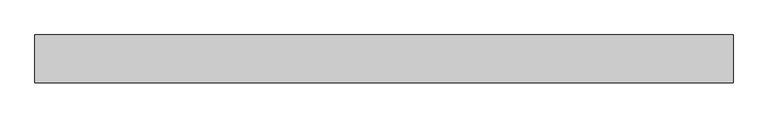
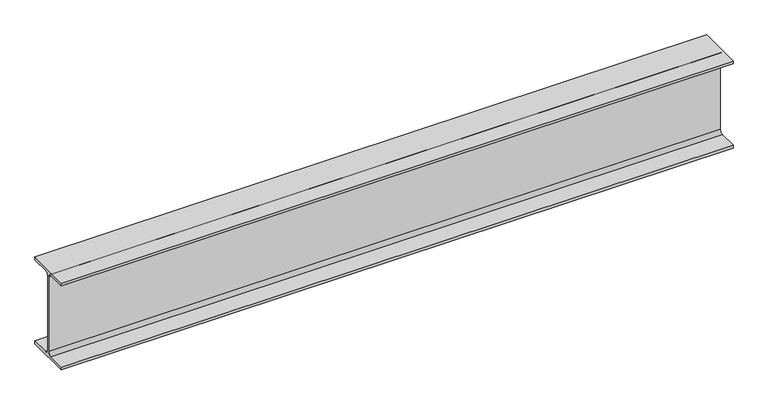
"""IFC4 building model written with IfcOpenShell, lengths in millimetres: beam geometry, 0912_Steel Framing_H-KSD3502 : H_SB_ASB_H-350x175x7x11."""

from ifc_helpers import new_model, si_unit, point, frame, frame_2d, origin, place, context, project, spatial, polyline, circle_curve, trimmed, segment, composite_curve, outline, extrude, source, transform, mapped, element, save


def beam_712d29b2(model_context):
    return source(origin(), model_context, "Body", "SweptSolid", [
        extrude(outline(composite_curve([segment(polyline([(87.5, -164.0), (87.5, -175.0), (-87.5, -175.0), (-87.5, -164.0), (-17.5, -164.0)]), True, "CONTINUOUS"), segment(trimmed(circle_curve(frame_2d((-17.5, -150.0)), 14.0), [point((-17.5, -164.0))], [point((-3.5, -150.0))], True, "CARTESIAN"), True, "CONTINUOUS"), segment(polyline([(-3.5, -150.0), (-3.5, 150.0)]), True, "CONTINUOUS"), segment(trimmed(circle_curve(frame_2d((-17.5, 150.0)), 14.0), [point((-3.5, 150.0))], [point((-17.5, 164.0))], True, "CARTESIAN"), True, "CONTINUOUS"), segment(polyline([(-17.5, 164.0), (-87.5, 164.0), (-87.5, 175.0), (87.5, 175.0), (87.5, 164.0), (17.5, 164.0)]), True, "CONTINUOUS"), segment(trimmed(circle_curve(frame_2d((17.5, 150.0)), 14.0), [point((17.5, 164.0))], [point((3.5, 150.0))], True, "CARTESIAN"), True, "CONTINUOUS"), segment(polyline([(3.5, 150.0), (3.5, -150.0)]), True, "CONTINUOUS"), segment(trimmed(circle_curve(frame_2d((17.5, -150.0)), 14.0), [point((3.5, -150.0))], [point((17.5, -164.0))], True, "CARTESIAN"), True, "CONTINUOUS"), segment(polyline([(17.5, -164.0), (87.5, -164.0)]), True, "CONTINUOUS")], self_intersect=False)), frame((-1265.9227894, 0.0, 0.0), z_axis=(1.0, 0.0, 0.0), x_axis=(0.0, 1.0, 0.0)), (0.0, 0.0, 1.0), 2561.6966945),
    ])


if __name__ == "__main__":
    model = new_model("IFC4")
    model_context = context("Model", 3, world=origin())
    ifc_project = project(units=[si_unit("LENGTHUNIT", "METRE", prefix="MILLI")], contexts=[model_context])
    site = spatial("IfcSite", under=ifc_project)
    building = spatial("IfcBuilding", under=site)
    placement = place(None, origin())
    beam_shape = beam_712d29b2(model_context)
    element("IfcBeam", 1, ObjectType="0912_Steel Framing_H-KSD3502 : H_SB_ASB_H-350x175x7x11", at=placement, inside=building, context=model_context, shape_type="MappedRepresentation", body=[
        mapped(beam_shape, transform((0.0, 0.0, 0.0), x_axis=(1.0, 0.0, 0.0), y_axis=(0.0, 1.0, 0.0), z_axis=(0.0, 0.0, 1.0))),
    ])
    save(model, "model.ifc")

# Revit data of these elements
# Type "0912_Steel Framing_H-KSD3502 : H_SB_ASB_H-350x175x7x11"
#   H_WM Code_1 = "S01AA002-00001 | Main Steel Structure Fabrication Work | Shelter/Building | Medium Steel - Standard (90KG/M>Weight≥30KG/M) | Material: (   )"
#   H_WM Code_2 = "S03AA028-00001 | Main Steel Structure Erection Work | Shelter/Building | Medium Steel (90KG/M>Weight≥30KG/M) | Material: (   )"
#   H_WM Code_3 = "S01AA010-00001 | Main Steel Structure Fabrication Work | Shelter/Building | Steel Painting/Coating | for Non-Fireproofed Steel Surface, Surface Preparation, Primer, Second & Final Coat | Material: (   )"
#   H_Q'ty Cal Type Tag = "SB-Q2"
#   Width = 17.5 cm
#   Web Thickness = 0.7 cm
#   Web Fillet = 1.4 cm
#   Warping Constant = 282000.0 cm⁶
#   W = 0
#   Torsional Moment of Inertia = 19.4042 cm⁴
#   Section Area = 63.14 cm²
#   Plastic Modulus weak axis = 174.0 cm³
#   Plastic Modulus strong axis = 868.0 cm³
#   Perimeter = 1.36 m²/m
#   Nominal Weight = 49.60 kgf/m
#   Moment of Inertia weak axis = 984.00 cm⁴
#   Moment of Inertia strong axis = 13600.00 cm⁴
#   Height = 35.0 cm
#   Flange Thickness = 1.1 cm
#   Elastic Modulus weak axis = 112.0 cm³
#   Elastic Modulus strong axis = 775.0 cm³
#   Centroid Vertical = 17.5 cm
#   Centroid Horizontal = 8.75 cm
#   Ix = 136000000
#   Length [instance default] = 1.5240 m
#   Zx = 868000
#   b = 0.1750 m
#   h = 0.3500 m
#   r = 0.0140 m
#   s = 0.0070 m
#   t = 0.0110 m
#   A = 0.006314 m²
#   Structural Material [instance default] = Steel, 45-345
#   Assembly Code = ""
# Element 1 (IfcBeam, "0912_Steel Framing_H-KSD3502 : H_SB_ASB_H-350x175x7x11")
#   Structural Material = none
# Materials
#   "Steel, 45-345": class "Metal", colour RGB 189 187 185, transparency 0, Description = "Steel 345 MPa", Cost = 0
